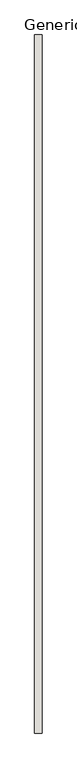
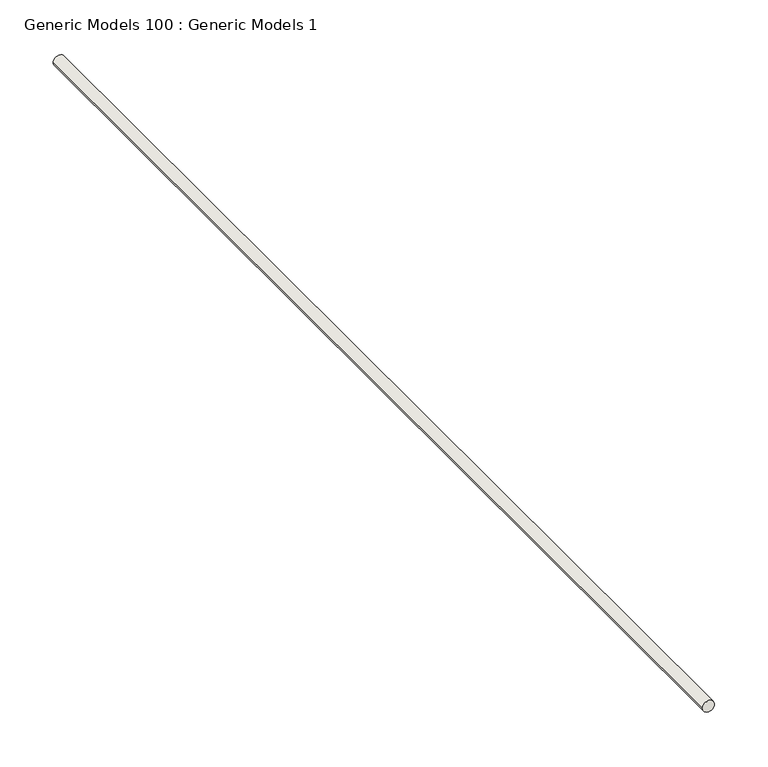
"""IFC4 building model written with IfcOpenShell, lengths in millimetres: wall geometry, Generic Models 100 : Generic Models 1."""

from ifc_helpers import new_model, si_unit, point, frame, frame_2d, origin, place, context, project, spatial, circle_curve, trimmed, segment, composite_curve, outline, extrude, source, transform, mapped, element, save


def generic_models_100_generic_models_1_345d56ba(model_context):
    return source(origin(), model_context, "Body", "SweptSolid", [
        extrude(outline(composite_curve([segment(trimmed(circle_curve(frame_2d((2085.43863, 376653.425)), 6.35), [point((2085.43863, 376647.075))], [point((2085.43863, 376659.775))], False, "CARTESIAN"), True, "CONTINUOUS"), segment(trimmed(circle_curve(frame_2d((2085.43863, 376653.425)), 6.35), [point((2085.43863, 376659.775))], [point((2085.43863, 376647.075))], False, "CARTESIAN"), True, "CONTINUOUS")], self_intersect=False)), frame((0.0, 76.2, 0.0), z_axis=(0.0, 1.0, 0.0), x_axis=(0.0, 0.0, 1.0)), (0.0, 0.0, 1.0), 1219.2),
    ])


if __name__ == "__main__":
    model = new_model("IFC4")
    model_context = context("Model", 3, world=origin())
    ifc_project = project(units=[si_unit("LENGTHUNIT", "METRE", prefix="MILLI")], contexts=[model_context])
    site = spatial("IfcSite", under=ifc_project)
    building = spatial("IfcBuilding", under=site)
    placement = place(None, origin())
    generic_models_100_generic_models_1_shape = generic_models_100_generic_models_1_345d56ba(model_context)
    element("IfcWall", 1, ObjectType="Generic Models 100 : Generic Models 1", at=placement, inside=building, context=model_context, shape_type="MappedRepresentation", body=[
        mapped(generic_models_100_generic_models_1_shape, transform((0.0, 0.0, 0.0), x_axis=(1.0, 0.0, 0.0), y_axis=(0.0, 1.0, 0.0), z_axis=(0.0, 0.0, 1.0))),
    ])
    save(model, "model.ifc")

# Revit data of these elements
# Element 1 (IfcWall, "Generic Models 100 : Generic Models 1")
#   Materials on its faces: "WALL REINFORCING - SEE PLAN SCHEDULES FOR SIZE/LOCATION"
# Materials
#   "WALL REINFORCING - SEE PLAN SCHEDULES FOR SIZE/LOCATION": class "Metal", colour RGB 189 187 185, transparency 0, Description = "Structural steel 50ksi", Cost = 0
